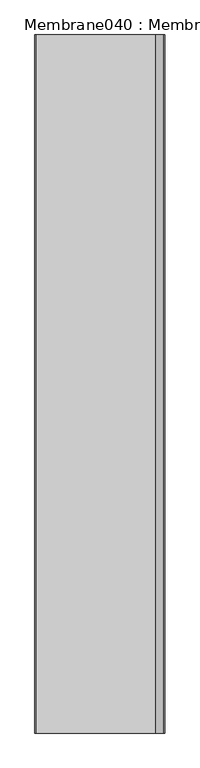
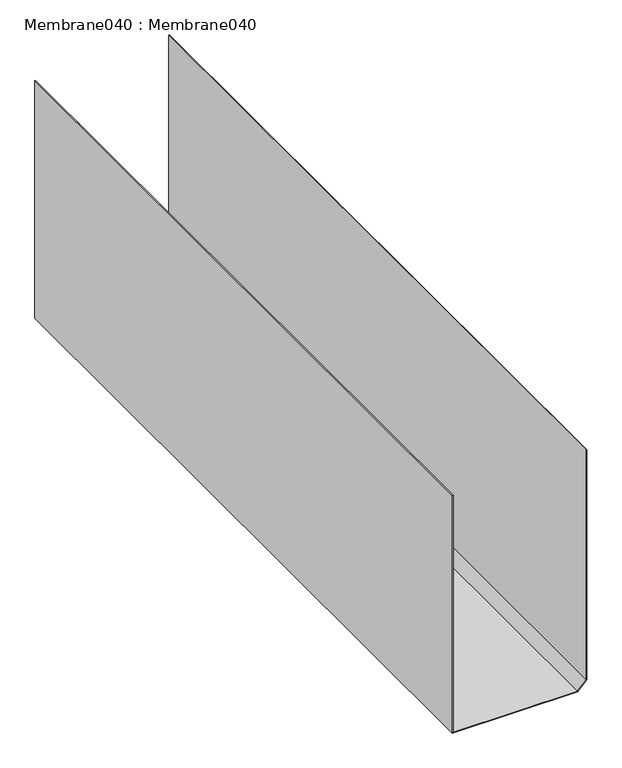
"""IFC4 building model written with IfcOpenShell, lengths in millimetres: proxy geometry, Membrane040 : Membrane040."""

import ifcopenshell
import ifcopenshell.guid

model = None  # the IFC model being written
_history = None  # IfcOwnerHistory: only IFC2X3 demands one
_inside = {}  # id of a spatial element -> (the spatial element, [elements in it])
_under = {}  # id of a project, library or spatial element -> (it, [spatial elements below it])
_declared = {}  # id of a project -> (the project, [libraries it declares])
_typed = {}  # id of a type object -> (the type object, [elements of that type])
_made_of = {}  # id of a material, layer set ... -> (it, [elements and type objects made of it])


def new_model(schema):
    """Start an empty IFC model of exactly this schema.

    Asked for "IFC4X3", IfcOpenShell would pick the latest addendum, in which some entities
    have other attributes; the version numbers below select the first issue.
    IFC2X3 requires an IfcOwnerHistory on every rooted entity: one is made here for all.
    """
    global model, _history
    if schema == "IFC4X3":
        model = ifcopenshell.file(schema_version=(4, 3, 0, 0))
    else:
        model = ifcopenshell.file(schema=schema)
    _inside.clear()
    _under.clear()
    _declared.clear()
    _typed.clear()
    _made_of.clear()
    _history = None
    if model.schema == "IFC2X3":
        org = make("IfcOrganization", Name="unknown")
        user = make(
            "IfcPersonAndOrganization",
            ThePerson=make("IfcPerson", FamilyName="unknown"),
            TheOrganization=org,
        )
        app = make(
            "IfcApplication",
            ApplicationDeveloper=org,
            Version="unknown",
            ApplicationFullName="unknown",
            ApplicationIdentifier="unknown",
        )
        _history = make(
            "IfcOwnerHistory",
            OwningUser=user,
            OwningApplication=app,
            ChangeAction="ADDED",
            CreationDate=0,
        )
    return model


def make(cls, **values):
    """One entity of the class cls with the attributes given. An attribute that is None is left unset."""
    return model.create_entity(
        cls, **{name: value for name, value in values.items() if value is not None}
    )


def rooted(cls, **values):
    """An entity with a GlobalId (a new one), such as an element, a storey or a relation."""
    return make(cls, GlobalId=ifcopenshell.guid.new(), OwnerHistory=_history, **values)


def si_unit(unit_type, name, prefix=None):
    """IfcSIUnit, for example si_unit("LENGTHUNIT", "METRE", prefix="MILLI")."""
    return make("IfcSIUnit", UnitType=unit_type, Prefix=prefix, Name=name)


def assignment(units):
    """IfcUnitAssignment: the units of a project."""
    return None if units is None else make("IfcUnitAssignment", Units=units)


def point(xyz):
    """IfcCartesianPoint."""
    return None if xyz is None else make("IfcCartesianPoint", Coordinates=xyz)


def direction(xyz):
    """IfcDirection."""
    return None if xyz is None else make("IfcDirection", DirectionRatios=xyz)


def frame(location, z_axis=None, x_axis=None):
    """IfcAxis2Placement3D, a coordinate frame: its origin and axes. An axis left out is left unset."""
    return make(
        "IfcAxis2Placement3D",
        Location=point(location),
        Axis=direction(z_axis),
        RefDirection=direction(x_axis),
    )


def origin():
    """The frame at (0, 0, 0) with its axes left unset."""
    return frame((0.0, 0.0, 0.0))


def place(relative_to, where):
    """IfcLocalPlacement: puts the frame where relative to a parent placement (None: the world)."""
    return make(
        "IfcLocalPlacement", PlacementRelTo=relative_to, RelativePlacement=where
    )


def context(
    kind, dimensions, precision=None, world=None, true_north=None, identifier=None
):
    """IfcGeometricRepresentationContext, for example the 3D "Model" context."""
    return make(
        "IfcGeometricRepresentationContext",
        ContextIdentifier=identifier,
        ContextType=kind,
        CoordinateSpaceDimension=dimensions,
        Precision=precision,
        WorldCoordinateSystem=world,
        TrueNorth=true_north,
    )


def project(units=None, contexts=None):
    """IfcProject with its units and contexts."""
    return rooted(
        "IfcProject",
        Name="project",
        RepresentationContexts=contexts,
        UnitsInContext=assignment(units),
    )


def spatial(cls, under=None, at=None, **own):
    """A site, building, storey or space (cls), placed at a placement, below another one or the project."""
    s = rooted(cls, ObjectPlacement=at, **own)
    if under is not None:
        _under.setdefault(under.id(), (under, []))[1].append(s)
    return s


def polyline(points):
    """IfcPolyline through the points."""
    return make("IfcPolyline", Points=[point(p) for p in points])


def outline(outer, holes=None, kind="AREA"):
    """IfcArbitraryClosedProfileDef: a profile drawn as a closed curve; with holes, ...WithVoids."""
    if holes is None:
        return make("IfcArbitraryClosedProfileDef", ProfileType=kind, OuterCurve=outer)
    return make(
        "IfcArbitraryProfileDefWithVoids",
        ProfileType=kind,
        OuterCurve=outer,
        InnerCurves=holes,
    )


def extrude(swept, where, along, depth):
    """IfcExtrudedAreaSolid: the profile swept, set in the frame where, extruded along a direction by depth."""
    return make(
        "IfcExtrudedAreaSolid",
        SweptArea=swept,
        Position=where,
        ExtrudedDirection=direction(along),
        Depth=depth,
    )


def shape(context_of_items, identifier, shape_type, items):
    """IfcShapeRepresentation: the items that make up one representation, for example the "Body"."""
    return make(
        "IfcShapeRepresentation",
        ContextOfItems=context_of_items,
        RepresentationIdentifier=identifier,
        RepresentationType=shape_type,
        Items=items,
    )


def source(mapping_origin, context_of_items, identifier, shape_type, items):
    """IfcRepresentationMap: a shape defined once, which mapped items show again and again."""
    return make(
        "IfcRepresentationMap",
        MappingOrigin=mapping_origin,
        MappedRepresentation=shape(context_of_items, identifier, shape_type, items),
    )


def transform(
    local_origin,
    x_axis=None,
    y_axis=None,
    z_axis=None,
    scale=None,
    scale2=None,
    scale3=None,
    uniform=True,
):
    """IfcCartesianTransformationOperator3D, or its non-uniform kind. x_axis, y_axis, z_axis: its Axis1, 2, 3."""
    if uniform:
        return make(
            "IfcCartesianTransformationOperator3D",
            Axis1=direction(x_axis),
            Axis2=direction(y_axis),
            LocalOrigin=point(local_origin),
            Scale=scale,
            Axis3=direction(z_axis),
        )
    return make(
        "IfcCartesianTransformationOperator3DnonUniform",
        Axis1=direction(x_axis),
        Axis2=direction(y_axis),
        LocalOrigin=point(local_origin),
        Scale=scale,
        Axis3=direction(z_axis),
        Scale2=scale2,
        Scale3=scale3,
    )


def mapped(mapping_source, mapping_target):
    """IfcMappedItem: shows the shape of a source again, moved by a transform."""
    return make(
        "IfcMappedItem", MappingSource=mapping_source, MappingTarget=mapping_target
    )


def made_of(thing, what):
    """Note that an element or type object is made of a material, layer set ...; save() writes the relation."""
    if what is not None:
        _made_of.setdefault(what.id(), (what, []))[1].append(thing)
    return thing


def element(
    cls,
    number,
    at=None,
    inside=None,
    cuts=None,
    type_object=None,
    material=None,
    context=None,
    identifier="Body",
    shape_type=None,
    held_by="IfcProductDefinitionShape",
    body=None,
    shapes=None,
    **own,
):
    """One element of the class cls, such as IfcWall. Its Tag is "e" and its number.

    at: its placement. inside: the storey or other place that contains it. cuts: it is an
    opening in that element (IfcRelVoidsElement). A single representation is given by context,
    identifier, shape_type and body (its items); several are given by shapes. held_by: the class
    of the entity that holds the representations. save() writes the other relations.
    """
    e = rooted(cls, Tag="e%d" % number, ObjectPlacement=at, **own)
    if body is not None:
        shapes = [shape(context, identifier, shape_type, body)]
    if shapes is not None:
        e.Representation = make(held_by, Representations=shapes)
    if inside is not None:
        _inside.setdefault(inside.id(), (inside, []))[1].append(e)
    if cuts is not None:
        rooted(
            "IfcRelVoidsElement", RelatingBuildingElement=cuts, RelatedOpeningElement=e
        )
    if type_object is not None:
        _typed.setdefault(type_object.id(), (type_object, []))[1].append(e)
    return made_of(e, material)


def aggregate(whole, parts):
    """IfcRelAggregates: a whole, such as a stair, and the parts it consists of."""
    return rooted("IfcRelAggregates", RelatingObject=whole, RelatedObjects=parts)


def save(model, path):
    """Write the relations noted so far, then the file.

    IfcRelAggregates (storeys below a building ...), IfcRelContainedInSpatialStructure (elements
    in a storey), IfcRelDefinesByType, IfcRelAssociatesMaterial and IfcRelDeclares: one each for
    every whole, place, type object, material and project.
    """
    for whole, parts in _under.values():
        aggregate(whole, parts)
    for where, things in _inside.values():
        rooted(
            "IfcRelContainedInSpatialStructure",
            RelatedElements=things,
            RelatingStructure=where,
        )
    for kind, things in _typed.values():
        rooted("IfcRelDefinesByType", RelatedObjects=things, RelatingType=kind)
    for what, things in _made_of.values():
        rooted("IfcRelAssociatesMaterial", RelatedObjects=things, RelatingMaterial=what)
    for by, libraries in _declared.values():
        rooted("IfcRelDeclares", RelatingContext=by, RelatedDefinitions=libraries)
    model.write(path)


def membrane040_membrane040_042d28cd(model_context):
    return source(origin(), model_context, "Body", "SweptSolid", [
        extrude(outline(polyline([(33312.9960937, -9692.7802734), (32641.4980103, -9692.7802734), (32616.7480469, -9716.9438184), (32616.7480469, -10060.5869141), (33309.0146212, -10060.5869141), (33309.0146212, -10062.5869141), (32614.7480469, -10062.5869141), (32614.7480469, -9716.101311), (32640.6835937, -9690.7802734), (33312.9960937, -9690.7802734), (33312.9960937, -9692.7802734)])), frame((0.0, 7982.1531721, 0.0), z_axis=(0.0, 1.0, 0.0), x_axis=(0.0, 0.0, 1.0)), (0.0, 0.0, 1.0), 2000.0),
    ])


if __name__ == "__main__":
    model = new_model("IFC4")
    model_context = context("Model", 3, world=origin())
    ifc_project = project(units=[si_unit("LENGTHUNIT", "METRE", prefix="MILLI")], contexts=[model_context])
    site = spatial("IfcSite", under=ifc_project)
    building = spatial("IfcBuilding", under=site)
    placement = place(None, origin())
    membrane040_membrane040_shape = membrane040_membrane040_042d28cd(model_context)
    element("IfcBuildingElementProxy", 1, Name="Membrane040 : Membrane040", ObjectType="Membrane040 : Membrane040", at=placement, inside=building, context=model_context, shape_type="MappedRepresentation", body=[
        mapped(membrane040_membrane040_shape, transform((0.0, 0.0, 0.0), x_axis=(1.0, 0.0, 0.0), y_axis=(0.0, 1.0, 0.0), z_axis=(0.0, 0.0, 1.0))),
    ])
    save(model, "model.ifc")

# Revit data of these elements
# Type "Membrane040 : Membrane040"
#   NameOverride = "Membrane040"
# Element 1 (IfcBuildingElementProxy, "Membrane040 : Membrane040")
#   Materials on its faces: "GEOTEXTILE FILTER FABRIC"
# Materials
#   "GEOTEXTILE FILTER FABRIC": class "Unassigned", colour RGB 254 255 135, transparency 0
